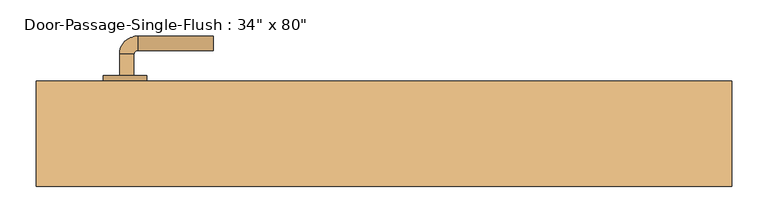
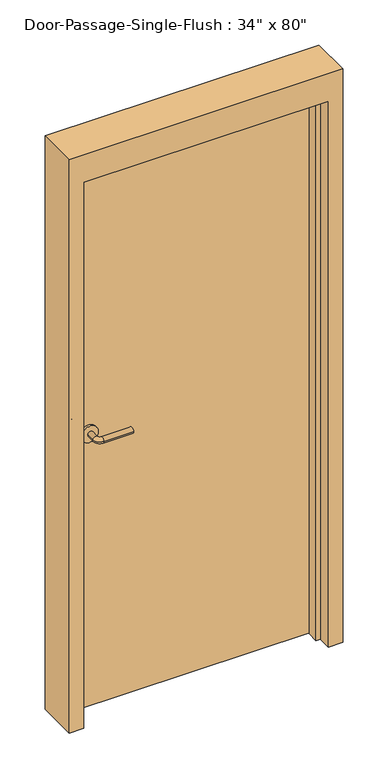
"""IFC4 building model written with IfcOpenShell, lengths in millimetres: door geometry."""

from ifc_helpers import new_model, si_unit, point, frame, frame_2d, origin, origin_with_axes, place, context, project, spatial, polyline, circle_curve, ellipse_curve, trimmed, segment, composite_curve, outline, extrude, faceted_brep, source, transform, mapped, element, save
from ifc_brep_helpers import plane_surface, cylinder_surface, revolved_surface, advanced_brep


def door_96787d45(model_context):
    return source(origin(), model_context, "Body", "SolidModel", [
        advanced_brep(
        [(-366.790625, 169.8, 1016.0), (-346.790625, 169.8, 1016.0), (-346.790625, 139.8, 1016.0), (-366.790625, 139.8, 1016.0), (-341.790625, 134.8, 1016.0), (-341.790625, 114.8, 1016.0), (-236.790625, 114.8, 1016.0), (-236.790625, 134.8, 1016.0)],
        [
            (0, 1, circle_curve(frame((-356.790625, 169.8, 1016.0), z_axis=(0.0, 1.0, 0.0), x_axis=(1.0, 0.0, 0.0)), 10.0)),
            (1, 0, circle_curve(frame((-356.790625, 169.8, 1016.0), z_axis=(0.0, 1.0, 0.0), x_axis=(1.0, 0.0, 0.0)), 10.0)),
            (1, 2),
            (2, 3, circle_curve(frame((-356.790625, 139.8, 1016.0), z_axis=(0.0, 1.0, 0.0), x_axis=(1.0, 0.0, 0.0)), 10.0)),
            (3, 0),
            (3, 2, circle_curve(frame((-356.790625, 139.8, 1016.0), z_axis=(0.0, 1.0, 0.0), x_axis=(1.0, 0.0, 0.0)), 10.0)),
            (4, 5, circle_curve(frame((-341.790625, 124.8, 1016.0), z_axis=(-1.0, 0.0, 0.0), x_axis=(0.0, 1.0, 0.0)), 10.0)),
            (5, 3, circle_curve(frame((-341.790625, 139.8, 1016.0), z_axis=(0.0, 0.0, -1.0), x_axis=(-1.0, 0.0, 0.0)), 25.0)),
            (2, 4, circle_curve(frame((-341.790625, 139.8, 1016.0), z_axis=(0.0, 0.0, 1.0), x_axis=(-1.0, 0.0, 0.0)), 5.0)),
            (5, 4, circle_curve(frame((-341.790625, 124.8, 1016.0), z_axis=(-1.0, 0.0, 0.0), x_axis=(0.0, 1.0, 0.0)), 10.0)),
            (6, 7, circle_curve(frame((-236.790625, 124.8, 1016.0), z_axis=(1.0, 0.0, 0.0), x_axis=(0.0, 1.0, 0.0)), 10.0)),
            (7, 6, circle_curve(frame((-236.790625, 124.8, 1016.0), z_axis=(1.0, 0.0, 0.0), x_axis=(0.0, 1.0, 0.0)), 10.0)),
            (4, 7),
            (6, 5),
        ],
        [
            plane_surface(frame((-356.790625, 169.8, 1016.0), z_axis=(0.0, 1.0, 0.0), x_axis=(0.0, 0.0, 1.0))),
            cylinder_surface(frame((-356.790625, 169.8, 1016.0), z_axis=(0.0, 1.0, 0.0), x_axis=(1.0, 0.0, 0.0)), 10.0),
            revolved_surface(trimmed(ellipse_curve(frame((-356.790625, 139.8, 1016.0), z_axis=(0.0, -1.0, 0.0), x_axis=(1.0, 0.0, 0.0)), 10.0, 10.0), [point((-366.790625, 139.8, 1016.0))], [point((-346.790625, 139.8, 1016.0))], True, "CARTESIAN"), (-341.790625, 139.8, 1016.0), (0.0, 0.0, -1.0)),
            revolved_surface(trimmed(ellipse_curve(frame((-356.790625, 139.8, 1016.0), z_axis=(0.0, -1.0, 0.0), x_axis=(1.0, 0.0, 0.0)), 10.0, 10.0), [point((-346.790625, 139.8, 1016.0))], [point((-366.790625, 139.8, 1016.0))], True, "CARTESIAN"), (-341.790625, 139.8, 1016.0), (0.0, 0.0, -1.0)),
            plane_surface(frame((-236.790625, 124.8, 1016.0), z_axis=(1.0, 0.0, 0.0), x_axis=(0.0, 0.0, 1.0))),
            cylinder_surface(frame((-341.790625, 124.8, 1016.0), z_axis=(-1.0, 0.0, 0.0), x_axis=(0.0, 1.0, 0.0)), 10.0),
        ],
        [
            (0, [[1, 2]]),
            (1, [[3, 4, 5, -2]]),
            (1, [[-5, 6, -3, -1]]),
            (2, [[7, 8, -4, 9]]),
            (3, [[10, -9, -6, -8]]),
            (4, [[11, 12]]),
            (5, [[13, -11, 14, -7]]),
            (5, [[-14, -12, -13, -10]]),
        ],
    ),
        extrude(outline(composite_curve([segment(trimmed(circle_curve(frame_2d((1016.0, -359.290625)), 30.0), [point((1016.0, -389.290625))], [point((1016.0, -329.290625))], False, "CARTESIAN"), True, "CONTINUOUS"), segment(trimmed(circle_curve(frame_2d((1016.0, -359.290625)), 30.0), [point((1016.0, -329.290625))], [point((1016.0, -389.290625))], False, "CARTESIAN"), True, "CONTINUOUS")], self_intersect=False)), frame((0.0, 169.8, 0.0), z_axis=(0.0, 1.0, 0.0), x_axis=(0.0, 0.0, 1.0)), (0.0, 0.0, 1.0), 8.0),
        advanced_brep(
        [(-366.790625, 236.6, 1016.0), (-346.790625, 236.6, 1016.0), (-366.790625, 266.6, 1016.0), (-346.790625, 266.6, 1016.0), (-341.790625, 271.6, 1016.0), (-341.790625, 291.6, 1016.0), (-236.790625, 291.6, 1016.0), (-236.790625, 271.6, 1016.0)],
        [
            (0, 1, circle_curve(frame((-356.790625, 236.6, 1016.0), z_axis=(0.0, -1.0, 0.0), x_axis=(1.0, 0.0, 0.0)), 10.0)),
            (1, 0, circle_curve(frame((-356.790625, 236.6, 1016.0), z_axis=(0.0, -1.0, 0.0), x_axis=(1.0, 0.0, 0.0)), 10.0)),
            (0, 2),
            (2, 3, circle_curve(frame((-356.790625, 266.6, 1016.0), z_axis=(0.0, -1.0, 0.0), x_axis=(1.0, 0.0, 0.0)), 10.0)),
            (3, 1),
            (3, 2, circle_curve(frame((-356.790625, 266.6, 1016.0), z_axis=(0.0, -1.0, 0.0), x_axis=(1.0, 0.0, 0.0)), 10.0)),
            (4, 3, circle_curve(frame((-341.790625, 266.6, 1016.0), z_axis=(0.0, 0.0, 1.0), x_axis=(-1.0, 0.0, 0.0)), 5.0)),
            (2, 5, circle_curve(frame((-341.790625, 266.6, 1016.0), z_axis=(0.0, 0.0, -1.0), x_axis=(-1.0, 0.0, 0.0)), 25.0)),
            (5, 4, circle_curve(frame((-341.790625, 281.6, 1016.0), z_axis=(-1.0, 0.0, 0.0), x_axis=(0.0, -1.0, 0.0)), 10.0)),
            (4, 5, circle_curve(frame((-341.790625, 281.6, 1016.0), z_axis=(-1.0, 0.0, 0.0), x_axis=(0.0, -1.0, 0.0)), 10.0)),
            (6, 7, circle_curve(frame((-236.790625, 281.6, 1016.0), z_axis=(1.0, 0.0, 0.0), x_axis=(0.0, -1.0, 0.0)), 10.0)),
            (7, 6, circle_curve(frame((-236.790625, 281.6, 1016.0), z_axis=(1.0, 0.0, 0.0), x_axis=(0.0, -1.0, 0.0)), 10.0)),
            (5, 6),
            (7, 4),
        ],
        [
            plane_surface(frame((-356.790625, 236.6, 1016.0), z_axis=(0.0, -1.0, 0.0), x_axis=(0.0, 0.0, 1.0))),
            cylinder_surface(frame((-356.790625, 236.6, 1016.0), z_axis=(0.0, -1.0, 0.0), x_axis=(1.0, 0.0, 0.0)), 10.0),
            revolved_surface(trimmed(ellipse_curve(frame((-356.790625, 266.6, 1016.0), z_axis=(0.0, -1.0, 0.0), x_axis=(1.0, 0.0, 0.0)), 10.0, 10.0), [point((-366.790625, 266.6, 1016.0))], [point((-346.790625, 266.6, 1016.0))], True, "CARTESIAN"), (-341.790625, 266.6, 1016.0), (0.0, 0.0, -1.0)),
            revolved_surface(trimmed(ellipse_curve(frame((-356.790625, 266.6, 1016.0), z_axis=(0.0, -1.0, 0.0), x_axis=(1.0, 0.0, 0.0)), 10.0, 10.0), [point((-346.790625, 266.6, 1016.0))], [point((-366.790625, 266.6, 1016.0))], True, "CARTESIAN"), (-341.790625, 266.6, 1016.0), (0.0, 0.0, -1.0)),
            plane_surface(frame((-236.790625, 281.6, 1016.0), z_axis=(1.0, 0.0, 0.0), x_axis=(0.0, 0.0, 1.0))),
            cylinder_surface(frame((-341.790625, 281.6, 1016.0), z_axis=(-1.0, 0.0, 0.0), x_axis=(0.0, -1.0, 0.0)), 10.0),
        ],
        [
            (0, [[1, 2]]),
            (1, [[-1, 3, 4, 5]]),
            (1, [[-2, -5, 6, -3]]),
            (2, [[7, -4, 8, 9]]),
            (3, [[-8, -6, -7, 10]]),
            (4, [[11, 12]]),
            (5, [[-9, 13, -12, 14]]),
            (5, [[-10, -14, -11, -13]]),
        ],
    ),
        extrude(outline(composite_curve([segment(trimmed(circle_curve(frame_2d((1016.0, -359.290625)), 30.0), [point((1016.0, -389.290625))], [point((1016.0, -329.290625))], False, "CARTESIAN"), True, "CONTINUOUS"), segment(trimmed(circle_curve(frame_2d((1016.0, -359.290625)), 30.0), [point((1016.0, -329.290625))], [point((1016.0, -389.290625))], False, "CARTESIAN"), True, "CONTINUOUS")], self_intersect=False)), frame((0.0, 228.6, 0.0), z_axis=(0.0, 1.0, 0.0), x_axis=(0.0, 0.0, 1.0)), (0.0, 0.0, 1.0), 8.0),
        faceted_brep([(431.8, 173.0375, 0.0), (431.8, 228.6, 0.0), (482.6, 228.6, 0.0), (482.6, 82.55, 0.0), (431.8, 82.55, 0.0), (431.8, 131.7625, 0.0), (415.925, 131.7625, 0.0), (415.925, 173.0375, 0.0), (431.8, 173.0375, 2032.0), (431.8, 228.6, 2032.0), (-431.8, 228.6, 2032.0), (-431.8, 228.6, 0.0), (-482.6, 228.6, 0.0), (-482.6, 228.6, 2133.6), (482.6, 228.6, 2133.6), (482.6, 82.55, 2133.6), (-482.6, 82.55, 2133.6), (-482.6, 82.55, 0.0), (-431.8, 82.55, 0.0), (-431.8, 82.55, 2032.0), (431.8, 82.55, 2032.0), (431.8, 131.7625, 2032.0), (-431.8, 131.7625, 2032.0), (-431.8, 131.7625, 0.0), (-415.925, 131.7625, 0.0), (-415.925, 131.7625, 2016.125), (415.925, 131.7625, 2016.125), (415.925, 173.0375, 2016.125), (-415.925, 173.0375, 2016.125), (-415.925, 173.0375, 0.0), (-431.8, 173.0375, 0.0), (-431.8, 173.0375, 2032.0)], [[[0, 1, 2, 3, 4, 5, 6, 7]], [[1, 0, 8, 9]], [[2, 1, 9, 10, 11, 12, 13, 14]], [[3, 2, 14, 15]], [[4, 3, 15, 16, 17, 18, 19, 20]], [[5, 4, 20, 21]], [[6, 5, 21, 22, 23, 24, 25, 26]], [[7, 6, 26, 27]], [[0, 7, 27, 28, 29, 30, 31, 8]], [[9, 8, 31, 10]], [[20, 19, 22, 21]], [[26, 25, 28, 27]], [[12, 11, 30, 29, 24, 23, 18, 17]], [[11, 10, 31, 30]], [[13, 12, 17, 16]], [[19, 18, 23, 22]], [[25, 24, 29, 28]], [[15, 14, 13, 16]]]),
        extrude(outline(polyline([(431.8, 177.8), (-431.8, 177.8), (-431.8, 228.6), (431.8, 228.6), (431.8, 177.8)])), origin_with_axes(), (0.0, 0.0, 1.0), 2032.0),
    ])


if __name__ == "__main__":
    model = new_model("IFC4")
    model_context = context("Model", 3, world=origin())
    ifc_project = project(units=[si_unit("LENGTHUNIT", "METRE", prefix="MILLI")], contexts=[model_context])
    site = spatial("IfcSite", under=ifc_project)
    building = spatial("IfcBuilding", under=site)
    placement = place(None, origin())
    door_shape = door_96787d45(model_context)
    element("IfcDoor", 1, ObjectType="Door-Passage-Single-Flush : 34\" x 80\"", at=placement, inside=building, context=model_context, shape_type="MappedRepresentation", body=[
        mapped(door_shape, transform((0.0, 0.0, 0.0), x_axis=(1.0, 0.0, 0.0), y_axis=(0.0, 1.0, 0.0), z_axis=(0.0, 0.0, 1.0))),
    ])
    save(model, "model.ifc")

# Revit data of these elements
# Type "Door-Passage-Single-Flush : 34\" x 80\""
#   Type Mark = "14"
#   Assembly Code = "C1020"
#   Analytic Construction = "Wooden"
#   Thickness = 0' - 2"
#   Thermal Resistance (R) = 2.5876 (h·ft²·°F)/BTU
#   Swing Angle [instance default] = 90.00°
#   Strike Height = 3' - 4"
#   Rough Width [instance default] = 3' - 2"
#   Rough Height [instance default] = 7' - 0"
#   Masonry Inset [instance default] = 0' - 1"
#   Masonry Frame Depth = 0' - 5 3/4"
#   MF Opening Width [instance default] = 0' - 4"
#   MF Opening Height [instance default] = 0' - 4"
#   Inset Calculate [instance default] = 0' - 4"
#   Heat Transfer Coefficient (U) = 0.3865 BTU/(h·ft²·°F)
#   Height = 6' - 8"
#   Width = 2' - 10"
#   Masonry Frame [instance default] = yes
#   Dry Wall Frame [instance default] = no
#   Panel Material = Wood - Birch
#   Door Handle Material = Aluminum
#   Frame Material = Door - Frame
#   Visual Light Transmittance = 0
#   Solar Heat Gain Coefficient = 0
#   Function = (empty or 0)
#   Wall Closure = (empty or 0)
# Element 1 (IfcDoor, "Door-Passage-Single-Flush : 34\" x 80\"")
#   Materials on its faces: "Aluminum", "Door - Frame", "Wood - Birch"
# Materials
#   "Wood - Birch": class "Unassigned", colour RGB 224 178 126, transparency 0
#   "Aluminum": class "Metal", colour RGB 244 244 244, transparency 0, Description = "Aluminum 6061", Cost = 0
#   "Door - Frame": class "Unassigned", colour RGB 118 70 51, transparency 0
